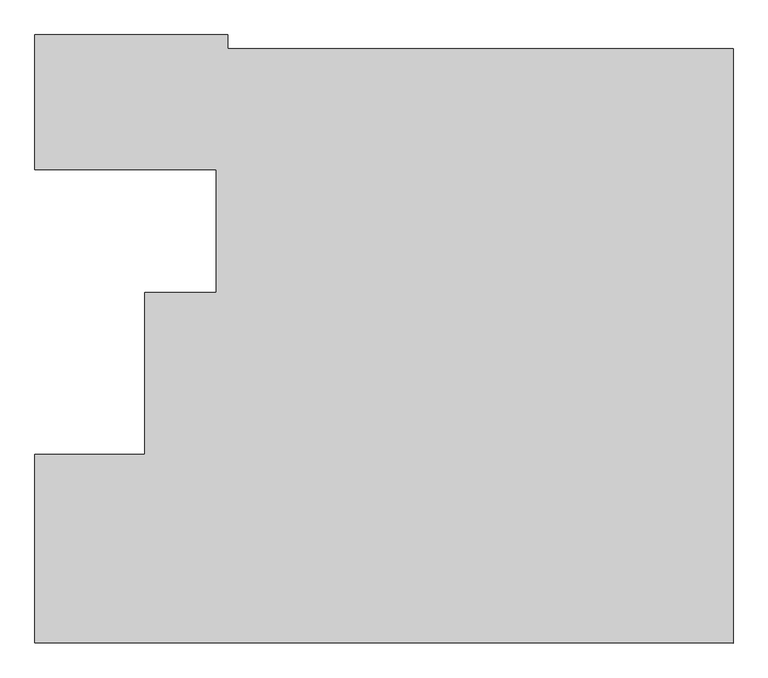
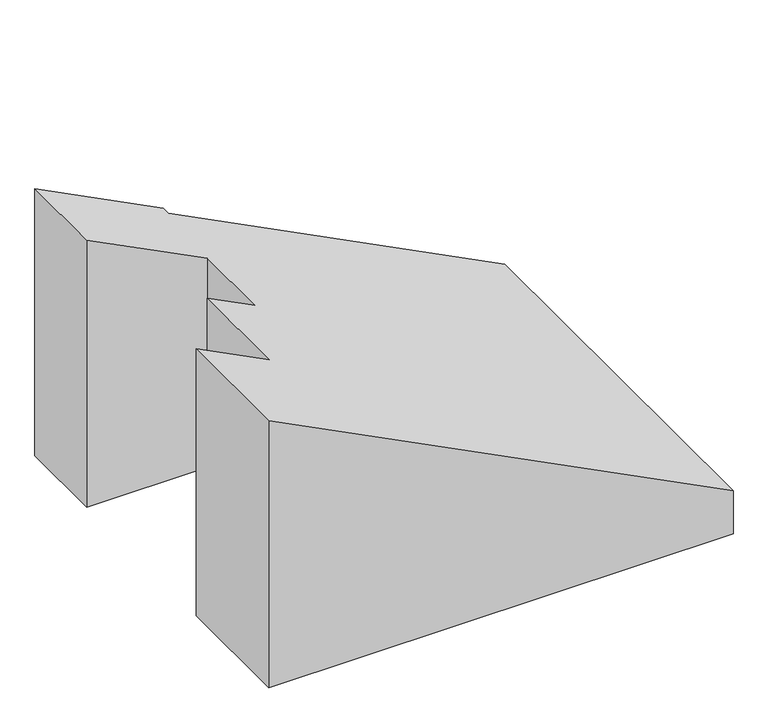
"""IFC4 building model written with IfcOpenShell, lengths in millimetres: proxy geometry, 0_3d."""

from ifc_helpers import new_model, si_unit, origin, place, context, project, spatial, faceted_brep, source, transform, mapped, element, save


def generic_models_ff5cb1ac(model_context):
    return source(origin(), model_context, "Body", "Brep", [
        faceted_brep([(1800.0, 5552.8619019, 3043.5797924), (1800.0, 5682.8619019, 3043.5797924), (0.0, 5682.8619019, 3960.7256015), (0.0, 4422.8619019, 3960.7256015), (1695.0, 4422.8619019, 3097.0799646), (1695.0, 3272.8619019, 3097.0799646), (1025.0, 3272.8619019, 3438.4620158), (1025.0, 1763.2600653, 3438.4620158), (0.0, 1763.2600653, 3960.7256015), (0.0, 0.0, 3960.7256015), (6520.0, 0.0, 638.6196708), (6520.0, 5552.8619019, 638.6196708), (1025.0, 3272.8619019, 0.0), (1025.0, 1763.2600653, 0.0), (1695.0, 3272.8619019, 0.0), (1695.0, 4422.8619019, 0.0), (0.0, 4422.8619019, 0.0), (1800.0, 5682.8619019, 0.0), (0.0, 5682.8619019, 0.0), (1800.0, 5552.8619019, 0.0), (6520.0, 5552.8619019, 0.0), (6520.0, 0.0, 0.0), (0.0, 0.0, 0.0), (0.0, 1763.2600653, 0.0)], [[[0, 1, 2, 3, 4, 5, 6, 7, 8, 9, 10, 11]], [[7, 6, 12, 13]], [[6, 5, 14, 12]], [[5, 4, 15, 14]], [[4, 3, 16, 15]], [[2, 1, 17, 18]], [[1, 0, 19, 17]], [[0, 11, 20, 19]], [[11, 10, 21, 20]], [[10, 9, 22, 21]], [[23, 22, 9, 8]], [[8, 7, 13, 23]], [[18, 16, 3, 2]], [[18, 17, 19, 20, 21, 22, 23, 13, 12, 14, 15, 16]]]),
    ])


if __name__ == "__main__":
    model = new_model("IFC4")
    model_context = context("Model", 3, world=origin())
    ifc_project = project(units=[si_unit("LENGTHUNIT", "METRE", prefix="MILLI")], contexts=[model_context])
    site = spatial("IfcSite", under=ifc_project)
    building = spatial("IfcBuilding", under=site)
    placement = place(None, origin())
    generic_models_shape = generic_models_ff5cb1ac(model_context)
    element("IfcBuildingElementProxy", 1, Name="0_3d", ObjectType="0_3d", at=placement, inside=building, context=model_context, shape_type="MappedRepresentation", body=[
        mapped(generic_models_shape, transform((0.0, 0.0, 0.0), x_axis=(1.0, 0.0, 0.0), y_axis=(0.0, 1.0, 0.0), z_axis=(0.0, 0.0, 1.0))),
    ])
    save(model, "model.ifc")

# Revit data of these elements
# Element 1 (IfcBuildingElementProxy, "0_3d")
#   Materials on its faces: "*1"
# Materials
#   "*1": class "Unassigned", colour RGB 175 175 175, transparency 0
